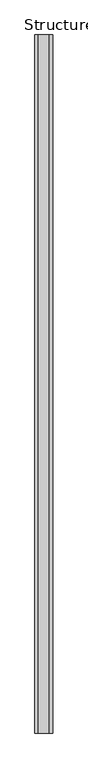
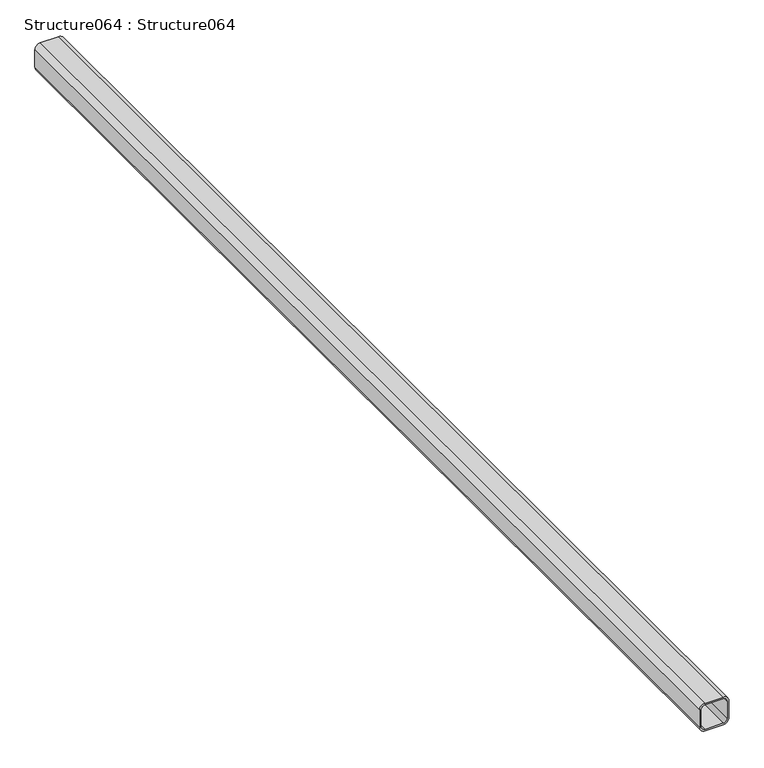
"""IFC4 building model written with IfcOpenShell, lengths in millimetres: proxy geometry, Structure064 : Structure064."""

from ifc_helpers import new_model, si_unit, point, frame, frame_2d, origin, place, context, project, spatial, polyline, circle_curve, trimmed, segment, composite_curve, outline, extrude, source, transform, mapped, element, save


def structure064_structure064_f60a5295(model_context):
    return source(origin(), model_context, "Body", "SweptSolid", [
        extrude(outline(composite_curve([segment(polyline([(40763.5716161, 16557.9969635), (40731.8216161, 16557.9969635)]), True, "CONTINUOUS"), segment(trimmed(circle_curve(frame_2d((40731.8216161, 16567.5219635)), 9.525), [point((40731.8216161, 16557.9969635))], [point((40722.2966161, 16567.5219635))], False, "CARTESIAN"), True, "CONTINUOUS"), segment(polyline([(40722.2966161, 16567.5219635), (40722.2966161, 16599.2719635)]), True, "CONTINUOUS"), segment(trimmed(circle_curve(frame_2d((40731.8216161, 16599.2719635)), 9.525), [point((40722.2966161, 16599.2719635))], [point((40731.8216161, 16608.7969635))], False, "CARTESIAN"), True, "CONTINUOUS"), segment(polyline([(40731.8216161, 16608.7969635), (40763.5716161, 16608.7969635)]), True, "CONTINUOUS"), segment(trimmed(circle_curve(frame_2d((40763.5716161, 16599.2719635)), 9.525), [point((40763.5716161, 16608.7969635))], [point((40773.0966161, 16599.2719635))], False, "CARTESIAN"), True, "CONTINUOUS"), segment(polyline([(40773.0966161, 16599.2719635), (40773.0966161, 16567.5219635)]), True, "CONTINUOUS"), segment(trimmed(circle_curve(frame_2d((40763.5716161, 16567.5219635)), 9.525), [point((40773.0966161, 16567.5219635))], [point((40763.5716161, 16557.9969635))], False, "CARTESIAN"), True, "CONTINUOUS")], self_intersect=False), holes=[composite_curve([segment(polyline([(40731.8216161, 16561.1719635), (40763.5716161, 16561.1719635)]), True, "CONTINUOUS"), segment(trimmed(circle_curve(frame_2d((40763.5716161, 16567.5219635)), 6.35), [point((40763.5716161, 16561.1719635))], [point((40769.9216161, 16567.5219635))], True, "CARTESIAN"), True, "CONTINUOUS"), segment(polyline([(40769.9216161, 16567.5219635), (40769.9216161, 16599.2719635)]), True, "CONTINUOUS"), segment(trimmed(circle_curve(frame_2d((40763.5716161, 16599.2719635)), 6.35), [point((40769.9216161, 16599.2719635))], [point((40763.5716161, 16605.6219635))], True, "CARTESIAN"), True, "CONTINUOUS"), segment(polyline([(40763.5716161, 16605.6219635), (40731.8216161, 16605.6219635)]), True, "CONTINUOUS"), segment(trimmed(circle_curve(frame_2d((40731.8216161, 16599.2719635)), 6.35), [point((40731.8216161, 16605.6219635))], [point((40725.4716161, 16599.2719635))], True, "CARTESIAN"), True, "CONTINUOUS"), segment(polyline([(40725.4716161, 16599.2719635), (40725.4716161, 16567.5219635)]), True, "CONTINUOUS"), segment(trimmed(circle_curve(frame_2d((40731.8216161, 16567.5219635)), 6.35), [point((40725.4716161, 16567.5219635))], [point((40731.8216161, 16561.1719635))], True, "CARTESIAN"), True, "CONTINUOUS")], self_intersect=False)]), frame((0.0, 7982.1449183, 0.0), z_axis=(0.0, 1.0, 0.0), x_axis=(0.0, 0.0, 1.0)), (0.0, 0.0, 1.0), 2000.0),
    ])


if __name__ == "__main__":
    model = new_model("IFC4")
    model_context = context("Model", 3, world=origin())
    ifc_project = project(units=[si_unit("LENGTHUNIT", "METRE", prefix="MILLI")], contexts=[model_context])
    site = spatial("IfcSite", under=ifc_project)
    building = spatial("IfcBuilding", under=site)
    placement = place(None, origin())
    structure064_structure064_shape = structure064_structure064_f60a5295(model_context)
    element("IfcBuildingElementProxy", 1, Name="Structure064 : Structure064", ObjectType="Structure064 : Structure064", at=placement, inside=building, context=model_context, shape_type="MappedRepresentation", body=[
        mapped(structure064_structure064_shape, transform((0.0, 0.0, 0.0), x_axis=(1.0, 0.0, 0.0), y_axis=(0.0, 1.0, 0.0), z_axis=(0.0, 0.0, 1.0))),
    ])
    save(model, "model.ifc")

# Revit data of these elements
# Type "Structure064 : Structure064"
#   NameOverride = "Structure064"
# Element 1 (IfcBuildingElementProxy, "Structure064 : Structure064")
#   Materials on its faces: "STEEL STRUCTURE (SEE STRUCTURAL DWGS)"
# Materials
#   "STEEL STRUCTURE (SEE STRUCTURAL DWGS)": class "Unassigned", colour RGB 128 128 128, transparency 0, Cost = 0
